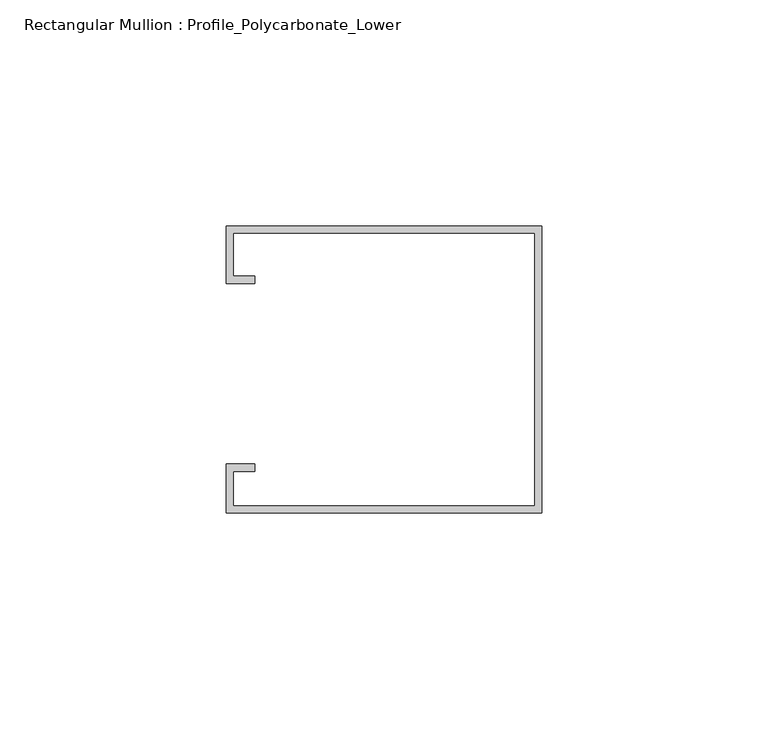
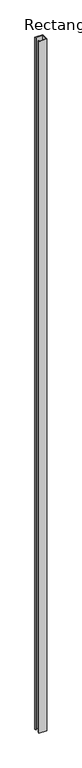
"""IFC4 building model written with IfcOpenShell, lengths in millimetres: member geometry, Rectangular Mullion : Profile_Polycarbonate_Lower."""

from ifc_helpers import new_model, si_unit, frame, origin, place, context, project, spatial, polyline, outline, extrude, source, transform, mapped, element, save


def rectangular_mullion_profile_polycarbonate_lower_8ae2b358(model_context):
    return source(origin(), model_context, "Body", "SweptSolid", [
        extrude(outline(polyline([(0.0, 32.7), (0.0, -30.8), (-69.85, -30.8), (-69.85, -20.0), (-63.5, -20.0), (-63.5, -21.5875), (-68.2625, -21.5875), (-68.2625, -29.2125), (-1.5875, -29.2125), (-1.5875, 31.1125), (-68.2625, 31.1125), (-68.2625, 21.5875), (-63.5, 21.5875), (-63.5, 20.0), (-69.85, 20.0), (-69.85, 32.7), (0.0, 32.7)])), frame((0.0, 0.0, -6565.9), z_axis=(0.0, 0.0, 1.0), x_axis=(1.0, 0.0, 0.0)), (0.0, 0.0, 1.0), 6565.9),
    ])


if __name__ == "__main__":
    model = new_model("IFC4")
    model_context = context("Model", 3, world=origin())
    ifc_project = project(units=[si_unit("LENGTHUNIT", "METRE", prefix="MILLI")], contexts=[model_context])
    site = spatial("IfcSite", under=ifc_project)
    building = spatial("IfcBuilding", under=site)
    placement = place(None, origin())
    rectangular_mullion_profile_polycarbonate_lower_shape = rectangular_mullion_profile_polycarbonate_lower_8ae2b358(model_context)
    element("IfcMember", 1, ObjectType="Rectangular Mullion : Profile_Polycarbonate_Lower", at=placement, inside=building, context=model_context, shape_type="MappedRepresentation", body=[
        mapped(rectangular_mullion_profile_polycarbonate_lower_shape, transform((0.0, 0.0, 0.0), x_axis=(1.0, 0.0, 0.0), y_axis=(0.0, 1.0, 0.0), z_axis=(0.0, 0.0, 1.0))),
    ])
    save(model, "model.ifc")

# Revit data of these elements
# Type "Rectangular Mullion : Profile_Polycarbonate_Lower"
#   built-in parameter 1007322 = 0.208333 (stored number, unit not read)
#   built-in parameter 1007321 = 0 (stored number, unit not read)
#   built-in parameter 1007320 = 0.00520833 (stored number, unit not read)
# Element 1 (IfcMember, "Rectangular Mullion : Profile_Polycarbonate_Lower")
#   Materials on its faces: "ALUMINUM PROFILE AT POLYCARBONATE PANEL"
# Materials
#   "ALUMINUM PROFILE AT POLYCARBONATE PANEL": class "Metal", colour RGB 244 244 244, transparency 0, Description = "Aluminum 6061", Cost = 0
